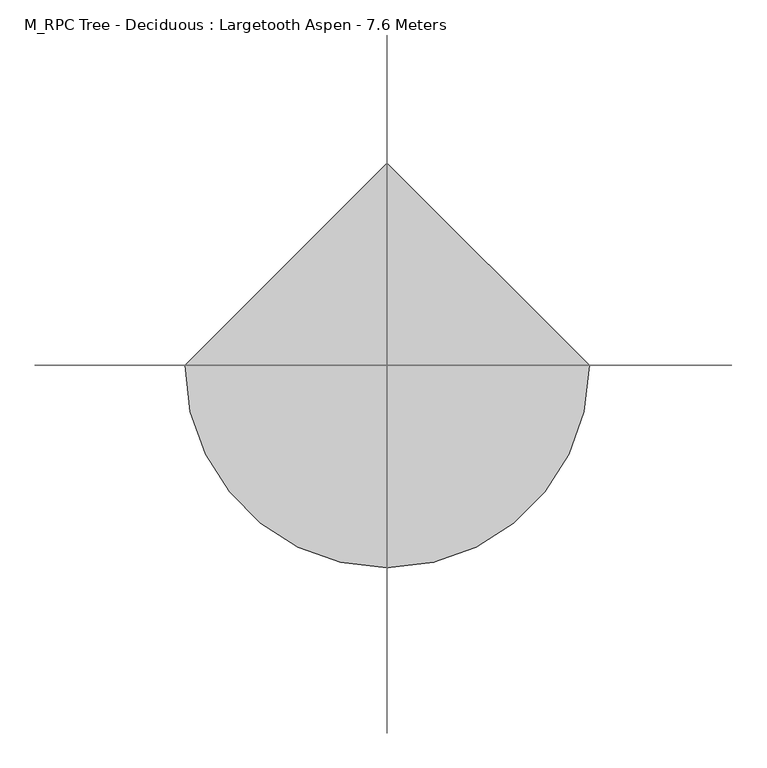
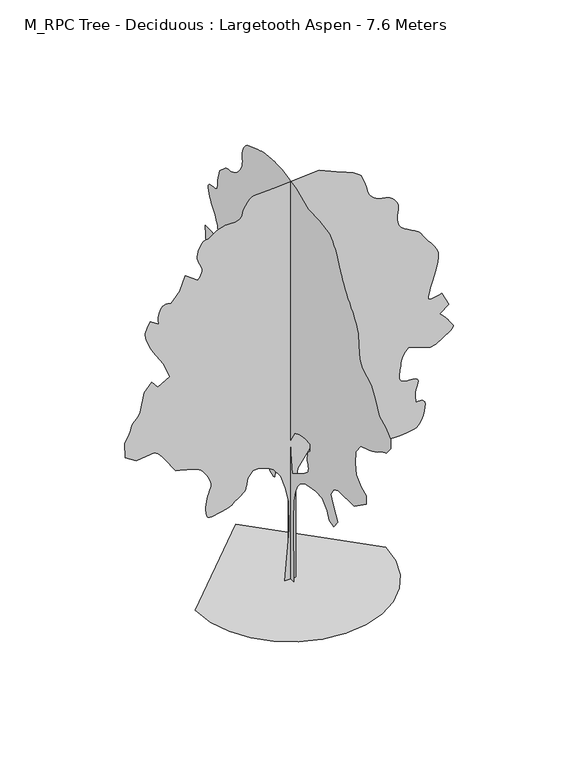
"""IFC4 building model written with IfcOpenShell, lengths in millimetres: geographic element geometry, M_RPC Tree - Deciduous : Largetooth Aspen - 7.6 Meters."""

import ifcopenshell
import ifcopenshell.guid

model = None  # the IFC model being written
_history = None  # IfcOwnerHistory: only IFC2X3 demands one
_inside = {}  # id of a spatial element -> (the spatial element, [elements in it])
_under = {}  # id of a project, library or spatial element -> (it, [spatial elements below it])
_declared = {}  # id of a project -> (the project, [libraries it declares])
_typed = {}  # id of a type object -> (the type object, [elements of that type])
_made_of = {}  # id of a material, layer set ... -> (it, [elements and type objects made of it])


def new_model(schema):
    """Start an empty IFC model of exactly this schema.

    Asked for "IFC4X3", IfcOpenShell would pick the latest addendum, in which some entities
    have other attributes; the version numbers below select the first issue.
    IFC2X3 requires an IfcOwnerHistory on every rooted entity: one is made here for all.
    """
    global model, _history
    if schema == "IFC4X3":
        model = ifcopenshell.file(schema_version=(4, 3, 0, 0))
    else:
        model = ifcopenshell.file(schema=schema)
    _inside.clear()
    _under.clear()
    _declared.clear()
    _typed.clear()
    _made_of.clear()
    _history = None
    if model.schema == "IFC2X3":
        org = make("IfcOrganization", Name="unknown")
        user = make(
            "IfcPersonAndOrganization",
            ThePerson=make("IfcPerson", FamilyName="unknown"),
            TheOrganization=org,
        )
        app = make(
            "IfcApplication",
            ApplicationDeveloper=org,
            Version="unknown",
            ApplicationFullName="unknown",
            ApplicationIdentifier="unknown",
        )
        _history = make(
            "IfcOwnerHistory",
            OwningUser=user,
            OwningApplication=app,
            ChangeAction="ADDED",
            CreationDate=0,
        )
    return model


def make(cls, **values):
    """One entity of the class cls with the attributes given. An attribute that is None is left unset."""
    return model.create_entity(
        cls, **{name: value for name, value in values.items() if value is not None}
    )


def rooted(cls, **values):
    """An entity with a GlobalId (a new one), such as an element, a storey or a relation."""
    return make(cls, GlobalId=ifcopenshell.guid.new(), OwnerHistory=_history, **values)


def si_unit(unit_type, name, prefix=None):
    """IfcSIUnit, for example si_unit("LENGTHUNIT", "METRE", prefix="MILLI")."""
    return make("IfcSIUnit", UnitType=unit_type, Prefix=prefix, Name=name)


def assignment(units):
    """IfcUnitAssignment: the units of a project."""
    return None if units is None else make("IfcUnitAssignment", Units=units)


def point(xyz):
    """IfcCartesianPoint."""
    return None if xyz is None else make("IfcCartesianPoint", Coordinates=xyz)


def direction(xyz):
    """IfcDirection."""
    return None if xyz is None else make("IfcDirection", DirectionRatios=xyz)


def frame(location, z_axis=None, x_axis=None):
    """IfcAxis2Placement3D, a coordinate frame: its origin and axes. An axis left out is left unset."""
    return make(
        "IfcAxis2Placement3D",
        Location=point(location),
        Axis=direction(z_axis),
        RefDirection=direction(x_axis),
    )


def origin():
    """The frame at (0, 0, 0) with its axes left unset."""
    return frame((0.0, 0.0, 0.0))


def place(relative_to, where):
    """IfcLocalPlacement: puts the frame where relative to a parent placement (None: the world)."""
    return make(
        "IfcLocalPlacement", PlacementRelTo=relative_to, RelativePlacement=where
    )


def context(
    kind, dimensions, precision=None, world=None, true_north=None, identifier=None
):
    """IfcGeometricRepresentationContext, for example the 3D "Model" context."""
    return make(
        "IfcGeometricRepresentationContext",
        ContextIdentifier=identifier,
        ContextType=kind,
        CoordinateSpaceDimension=dimensions,
        Precision=precision,
        WorldCoordinateSystem=world,
        TrueNorth=true_north,
    )


def project(units=None, contexts=None):
    """IfcProject with its units and contexts."""
    return rooted(
        "IfcProject",
        Name="project",
        RepresentationContexts=contexts,
        UnitsInContext=assignment(units),
    )


def spatial(cls, under=None, at=None, **own):
    """A site, building, storey or space (cls), placed at a placement, below another one or the project."""
    s = rooted(cls, ObjectPlacement=at, **own)
    if under is not None:
        _under.setdefault(under.id(), (under, []))[1].append(s)
    return s


def point_list(points):
    """IfcCartesianPointList2D or 3D."""
    cls = (
        "IfcCartesianPointList2D" if len(points[0]) == 2 else "IfcCartesianPointList3D"
    )
    return make(cls, CoordList=points)


def triangles(points, corners, closed=None, point_numbers=None):
    """IfcTriangulatedFaceSet: each triangle names its three corners, points numbered from 1."""
    return make(
        "IfcTriangulatedFaceSet",
        Coordinates=point_list(points),
        Closed=closed,
        CoordIndex=corners,
        PnIndex=point_numbers,
    )


def shape(context_of_items, identifier, shape_type, items):
    """IfcShapeRepresentation: the items that make up one representation, for example the "Body"."""
    return make(
        "IfcShapeRepresentation",
        ContextOfItems=context_of_items,
        RepresentationIdentifier=identifier,
        RepresentationType=shape_type,
        Items=items,
    )


def source(mapping_origin, context_of_items, identifier, shape_type, items):
    """IfcRepresentationMap: a shape defined once, which mapped items show again and again."""
    return make(
        "IfcRepresentationMap",
        MappingOrigin=mapping_origin,
        MappedRepresentation=shape(context_of_items, identifier, shape_type, items),
    )


def transform(
    local_origin,
    x_axis=None,
    y_axis=None,
    z_axis=None,
    scale=None,
    scale2=None,
    scale3=None,
    uniform=True,
):
    """IfcCartesianTransformationOperator3D, or its non-uniform kind. x_axis, y_axis, z_axis: its Axis1, 2, 3."""
    if uniform:
        return make(
            "IfcCartesianTransformationOperator3D",
            Axis1=direction(x_axis),
            Axis2=direction(y_axis),
            LocalOrigin=point(local_origin),
            Scale=scale,
            Axis3=direction(z_axis),
        )
    return make(
        "IfcCartesianTransformationOperator3DnonUniform",
        Axis1=direction(x_axis),
        Axis2=direction(y_axis),
        LocalOrigin=point(local_origin),
        Scale=scale,
        Axis3=direction(z_axis),
        Scale2=scale2,
        Scale3=scale3,
    )


def mapped(mapping_source, mapping_target):
    """IfcMappedItem: shows the shape of a source again, moved by a transform."""
    return make(
        "IfcMappedItem", MappingSource=mapping_source, MappingTarget=mapping_target
    )


def made_of(thing, what):
    """Note that an element or type object is made of a material, layer set ...; save() writes the relation."""
    if what is not None:
        _made_of.setdefault(what.id(), (what, []))[1].append(thing)
    return thing


def element(
    cls,
    number,
    at=None,
    inside=None,
    cuts=None,
    type_object=None,
    material=None,
    context=None,
    identifier="Body",
    shape_type=None,
    held_by="IfcProductDefinitionShape",
    body=None,
    shapes=None,
    **own,
):
    """One element of the class cls, such as IfcWall. Its Tag is "e" and its number.

    at: its placement. inside: the storey or other place that contains it. cuts: it is an
    opening in that element (IfcRelVoidsElement). A single representation is given by context,
    identifier, shape_type and body (its items); several are given by shapes. held_by: the class
    of the entity that holds the representations. save() writes the other relations.
    """
    e = rooted(cls, Tag="e%d" % number, ObjectPlacement=at, **own)
    if body is not None:
        shapes = [shape(context, identifier, shape_type, body)]
    if shapes is not None:
        e.Representation = make(held_by, Representations=shapes)
    if inside is not None:
        _inside.setdefault(inside.id(), (inside, []))[1].append(e)
    if cuts is not None:
        rooted(
            "IfcRelVoidsElement", RelatingBuildingElement=cuts, RelatedOpeningElement=e
        )
    if type_object is not None:
        _typed.setdefault(type_object.id(), (type_object, []))[1].append(e)
    return made_of(e, material)


def aggregate(whole, parts):
    """IfcRelAggregates: a whole, such as a stair, and the parts it consists of."""
    return rooted("IfcRelAggregates", RelatingObject=whole, RelatedObjects=parts)


def save(model, path):
    """Write the relations noted so far, then the file.

    IfcRelAggregates (storeys below a building ...), IfcRelContainedInSpatialStructure (elements
    in a storey), IfcRelDefinesByType, IfcRelAssociatesMaterial and IfcRelDeclares: one each for
    every whole, place, type object, material and project.
    """
    for whole, parts in _under.values():
        aggregate(whole, parts)
    for where, things in _inside.values():
        rooted(
            "IfcRelContainedInSpatialStructure",
            RelatedElements=things,
            RelatingStructure=where,
        )
    for kind, things in _typed.values():
        rooted("IfcRelDefinesByType", RelatedObjects=things, RelatingType=kind)
    for what, things in _made_of.values():
        rooted("IfcRelAssociatesMaterial", RelatedObjects=things, RelatingMaterial=what)
    for by, libraries in _declared.values():
        rooted("IfcRelDeclares", RelatingContext=by, RelatedDefinitions=libraries)
    model.write(path)


def m_rpc_tree_deciduous_largetooth_aspen_7_6_meters_a2efc43f(model_context):
    return source(origin(), model_context, "Body", "Tessellation", [
        triangles([(92.8617737, 0.000406, 0.005513), (-103.915959, 0.000406, 0.005513), (-22.8901635, 0.0003494, 949.1680813), (-34.4652064, 0.0003176, 1481.626133), (-92.3406663, 0.0003011, 1759.4311237), (-173.3674883, 0.0002866, 2002.5093098), (-300.6936918, 0.0002762, 2176.1362118), (-404.8693279, 0.0002728, 2234.0127663), (-566.9214277, 0.0002694, 2291.8891754), (-682.6743914, 0.0002694, 2291.8891754), (-763.7004049, 0.0002762, 2176.1362118), (-798.427355, 0.0002852, 2025.6589142), (-801.2950579, 0.0002863, 2008.1460297), (-806.4934324, 0.0002874, 1989.7185207), (-816.3455927, 0.0002886, 1969.4722275), (-833.1871519, 0.0002899, 1946.489764), (-859.3387533, 0.0002915, 1919.8644997), (-897.1360102, 0.0002934, 1888.6816647), (-948.9046526, 0.0002956, 1852.0320122), (-998.3097038, 0.0002977, 1817.003627), (-1032.3247061, 0.0002993, 1790.0718407), (-1058.2431822, 0.0003005, 1769.4200489), (-1083.3510246, 0.0003015, 1753.2219097), (-1114.9365967, 0.0003023, 1739.6560226), (-1160.2933485, 0.000303, 1726.8980804), (-1226.7072453, 0.0003038, 1713.1294441), (-1299.8367931, 0.0003048, 1697.5064152), (-1361.0192505, 0.0003056, 1683.0943588), (-1411.0653236, 0.0003062, 1673.9514576), (-1450.7852829, 0.0003062, 1674.1187439), (-1480.9902706, 0.0003054, 1687.6517841), (-1502.4856155, 0.0003035, 1718.5964069), (-1516.0869656, 0.0003004, 1771.0059986), (-1522.0251205, 0.0002967, 1833.4043701), (-1521.0802654, 0.0002932, 1891.7521168), (-1514.8710514, 0.00029, 1946.2541679), (-1505.0164204, 0.0002869, 1997.1108021), (-1493.1376396, 0.0002841, 2044.5246231), (-1480.8535057, 0.0002815, 2088.6983803), (-1469.7852859, 0.000279, 2129.8370029), (-1458.1775642, 0.0002769, 2165.8103886), (-1444.9485752, 0.000275, 2196.5194153), (-1432.7328964, 0.0002733, 2225.2042923), (-1424.1600185, 0.0002715, 2255.1052288), (-1421.8648098, 0.0002695, 2289.4596725), (-1428.479377, 0.000267, 2331.5079781), (-1446.6356815, 0.0002638, 2384.4900639), (-1473.3978561, 0.0002604, 2441.7913628), (-1503.3976238, 0.0002573, 2494.2338013), (-1535.6266159, 0.0002545, 2541.2094223), (-1569.0690514, 0.0002521, 2582.1226227), (-1602.7142361, 0.00025, 2616.3228607), (-1635.5487144, 0.0002484, 2643.2520309), (-1666.5642632, 0.0002473, 2662.3026123), (-1701.7269424, 0.0002464, 2677.1732162), (-1746.6125748, 0.0002455, 2692.0694), (-1799.5946606, 0.0002446, 2706.940004), (-1859.0568741, 0.0002437, 2721.8358971), (-1923.3782387, 0.0002428, 2736.706501), (-1990.9396671, 0.000242, 2751.5771049), (-2060.1197468, 0.0002411, 2766.4732887), (-2256.8962532, 0.0002238, 3055.8556252), (-2301.7818855, 0.0002202, 3116.5289566), (-2338.160479, 0.0002175, 3161.4195305), (-2367.4508423, 0.0002156, 3193.1367805), (-2391.0741096, 0.0002144, 3214.3154297), (-2410.4440029, 0.0002136, 3227.61549), (-2426.9815109, 0.0002131, 3235.6461044), (-2442.1003555, 0.0002128, 3241.041996), (-2766.1945267, 0.0002148, 3206.3353935), (-2962.9836777, 0.0002073, 3333.6607613), (-2974.5611687, 0.0001914, 3599.8884064), (-2952.3436295, 0.000189, 3639.5351143), (-2930.8609291, 0.0001867, 3678.9789276), (-2910.7717484, 0.0001843, 3718.0428223), (-2892.8103447, 0.0001821, 3756.473616), (-2877.7118477, 0.0001798, 3794.0934128), (-2866.1343567, 0.0001776, 3830.70019), (-2858.8130013, 0.0001755, 3866.1160515), (-2847.3878265, 0.0001735, 3899.5814507), (-2825.6772331, 0.0001716, 3931.2481224), (-2797.4559906, 0.0001698, 3962.0787987), (-2766.6000252, 0.0001679, 3993.137368), (-2736.9852631, 0.000166, 4025.3865623), (-2712.4120537, 0.000164, 4059.8905609), (-2696.7560326, 0.0001617, 4097.611805), (-2627.2919586, 0.000141, 4444.881015), (-2488.4021805, 0.0001321, 4595.3354942), (-2384.2239464, 0.0001396, 4468.0101265), (-2164.2953648, 0.0001327, 4583.7832924), (-2280.0483284, 0.0001155, 4873.1403397), (-2465.2501053, 9.82e-05, 5162.5226761), (-2487.5231644, 9.58e-05, 5203.6643509), (-2513.036142, 9.27e-05, 5254.9385468), (-2539.3601166, 8.93e-05, 5312.268187), (-2564.0600624, 8.58e-05, 5371.6238663), (-2584.7067673, 8.24e-05, 5428.9535065), (-2598.8934013, 7.93e-05, 5480.2277023), (-2604.1628471, 7.69e-05, 5521.3693771), (-2601.4519661, 7.48e-05, 5555.7463486), (-2593.9027176, 7.28e-05, 5589.5407974), (-2582.2746483, 7.08e-05, 5622.8038834), (-2567.4293335, 6.89e-05, 5655.6611801), (-2550.1521904, 6.69e-05, 5688.2394241), (-2531.2585762, 6.5e-05, 5720.5903564), (-2511.5516396, 6.31e-05, 5752.8651306), (-2361.0744873, 6.93e-05, 5648.6941635), (-2365.8675087, 6.73e-05, 5681.019516), (-2369.6472198, 6.54e-05, 5713.8518143), (-2371.4003105, 6.34e-05, 5747.6968414), (-2370.118412, 6.13e-05, 5783.0621246), (-2364.7857433, 5.9e-05, 5820.4540283), (-2354.391465, 5.67e-05, 5860.3794983), (-2337.9248829, 5.41e-05, 5903.344899), (-2316.394075, 5.19e-05, 5940.9141174), (-2291.8258072, 5.04e-05, 5965.7155106), (-2264.7267345, 4.95e-05, 5979.8768555), (-2235.6036575, 4.92e-05, 5985.5515091), (-2204.9604698, 4.92e-05, 5984.8422501), (-2173.3064426, 4.95e-05, 5979.8768555), (-2141.1459057, 5e-05, 5972.7831024), (-1990.6686081, 3.96e-05, 6146.4178528), (-1886.4928448, 2.44e-05, 6401.0680069), (-1666.5642632, 3.41e-05, 6239.0110382), (-1644.4939533, 3.23e-05, 6268.8284042), (-1623.9409927, 3.05e-05, 6298.823085), (-1606.4256374, 2.87e-05, 6329.2229736), (-1593.4675621, 2.69e-05, 6360.2309647), (-1586.584552, 2.5e-05, 6392.0749512), (-1587.2913403, 2.3e-05, 6424.9066681), (-1597.1131245, 2.1e-05, 6458.9545898), (-1613.1085144, 1.89e-05, 6493.7879288), (-1630.1173599, 1.68e-05, 6529.2043716), (-1646.3153538, 1.46e-05, 6565.8614365), (-1659.8813862, 1.23e-05, 6604.3428085), (-1668.993766, 9.9e-06, 6645.2304291), (-1671.8286221, 7.3e-06, 6689.1585617), (-1666.5642632, 4.4e-06, 6736.759726), (-1653.9432312, 1.5e-06, 6785.3747818), (-1636.4607227, -1.2e-06, 6830.974324), (-1614.9299149, -3.6e-06, 6871.9131042), (-1590.1616592, -5.7e-06, 6906.5691284), (-1562.9612846, -7.3e-06, 6933.3209839), (-1534.1394974, -8.3e-06, 6950.5728378), (-1504.512236, -8.7e-06, 6956.6782791), (-1471.3382435, -9.2e-06, 6965.0132355), (-1431.8891979, -1.05e-05, 6986.521225), (-1386.9707188, -1.22e-05, 7015.9078033), (-1337.3959831, -1.41e-05, 7047.9291046), (-1283.9756973, -1.59e-05, 7077.315683), (-1227.5178062, -1.72e-05, 7098.8236725), (-1168.8306908, -1.77e-05, 7107.1580475), (-1109.0314339, -1.76e-05, 7106.8289978), (-1050.4481638, -1.77e-05, 7107.2847839), (-995.7104439, -1.79e-05, 7110.8060806), (-947.4530697, -1.84e-05, 7119.5718246), (-908.3054592, -1.94e-05, 7135.8353668), (-880.9024807, -2.09e-05, 7161.8273849), (-867.8760956, -2.32e-05, 7199.7512329), (-856.9422426, -2.61e-05, 7248.5941818), (-835.6824938, -2.93e-05, 7302.6804153), (-806.5264246, -3.26e-05, 7357.4009125), (-771.9008492, -3.56e-05, 7408.0420074), (-734.2403572, -3.81e-05, 7449.9940979), (-695.9718355, -3.98e-05, 7478.5696793), (-659.5247869, -4.04e-05, 7489.1335693), (-323.8458215, -4.18e-05, 7512.2885513), (509.5693688, -4.53e-05, 7570.1751343), (926.2744205, -3.42e-05, 7384.9631836), (995.3532709, -3.26e-05, 7357.5526474), (1062.2078384, -3.09e-05, 7329.4578506), (1124.6038118, -2.92e-05, 7299.9195374), (1180.3219225, -2.73e-05, 7268.2778641), (1227.1277138, -2.52e-05, 7233.7741562), (1262.7970482, -2.29e-05, 7195.7485703), (1285.1055702, -2.04e-05, 7153.4674301), (1299.9533558, -1.79e-05, 7111.9461273), (1314.5985374, -1.58e-05, 7075.1117477), (1328.8409821, -1.37e-05, 7040.480722), (1342.4753242, -1.16e-05, 7005.6473831), (1355.2991055, -9.4e-06, 6968.1799026), (1367.1094311, -6.8e-06, 6925.6702881), (1377.7063133, -3.9e-06, 6875.662294), (1393.5345623, -8e-07, 6823.9573105), (1419.2834267, 2e-06, 6778.1292938), (1452.117905, 4.3e-06, 6738.3811386), (1489.2059029, 6.3e-06, 6704.890741), (1527.709948, 7.9e-06, 6677.9104111), (1564.7979458, 9.1e-06, 6657.5936279), (1597.6348949, 9.9e-06, 6644.1415421), (1628.0070236, 1.04e-05, 6636.0856384), (1659.1872425, 1.07e-05, 6630.6638763), (1690.5726814, 1.1e-05, 6626.230426), (1721.5527672, 1.13e-05, 6621.2144531), (1751.5195427, 1.17e-05, 6613.9439667), (1779.8675217, 1.24e-05, 6602.8481323), (1805.9861309, 1.34e-05, 6586.2799576), (1831.2638031, 1.47e-05, 6563.7586578), (1856.5388592, 1.63e-05, 6536.6015945), (1880.3977226, 1.82e-05, 6505.7959167), (1901.4218754, 2.02e-05, 6472.3560974), (1918.1949795, 2.23e-05, 6437.2948654), (1929.2986622, 2.44e-05, 6401.625531), (1933.3139694, 2.65e-05, 6366.3364059), (1929.8053173, 2.9e-05, 6325.1191544), (1922.2457497, 3.2e-05, 6273.1351181), (1915.0916805, 3.56e-05, 6213.8805954), (1912.7964718, 3.93e-05, 6150.775145), (1919.8163921, 4.31e-05, 6087.2644867), (1940.6048035, 4.67e-05, 6026.7937592), (1979.615649, 5e-05, 5972.7831024), (2034.2165314, 5.26e-05, 5927.5631882), (2096.1082478, 5.5e-05, 5888.8289246), (2161.2401733, 5.71e-05, 5853.1340103), (2225.5615379, 5.92e-05, 5817.0088898), (2285.0238968, 6.16e-05, 5777.0584213), (2335.5764797, 6.44e-05, 5729.8118866), (2373.1711327, 6.79e-05, 5671.8491455), (2411.6421856, 7.17e-05, 5607.223439), (2462.6659607, 7.56e-05, 5541.7878983), (2518.9567108, 7.96e-05, 5474.7303635), (2573.2307236, 8.38e-05, 5405.2410004), (2618.1721664, 8.81e-05, 5332.5093933), (2646.5201454, 9.27e-05, 5255.7495438), (2650.9785942, 9.76e-05, 5174.0998764), (2634.6386032, 0.0001032, 5079.7841217), (2608.190799, 0.0001097, 4970.8762344), (2575.6628426, 0.0001165, 4855.508567), (2541.0826859, 0.0001233, 4741.7367325), (2508.5622871, 0.0001295, 4637.6927925), (2482.1043091, 0.0001347, 4551.4835197), (2465.7718758, 0.0001383, 4491.1648178), (2464.9611694, 0.0001404, 4454.9635391), (2480.5538223, 0.0001417, 4433.9369156), (2509.8113388, 0.0001422, 4425.5769608), (2550.0001648, 0.0001421, 4427.3248192), (2598.3867462, 0.0001415, 4436.6727951), (2652.2453773, 0.0001407, 4451.0876129), (2708.839888, 0.0001396, 4468.0101265), (2836.1652557, 0.0001548, 4213.3596817), (2674.1332855, 0.0001624, 4086.0346046), (2698.8841003, 0.0001637, 4063.6400414), (2723.4573097, 0.0001651, 4040.7132431), (2747.6253113, 0.0001665, 4016.7987144), (2771.1852104, 0.0001681, 3991.3386406), (2793.9344032, 0.0001697, 3963.8772354), (2815.6705765, 0.0001715, 3933.8828453), (2836.1652557, 0.0001735, 3900.8482338), (2858.1037422, 0.0001754, 3868.6749069), (2881.2584335, 0.000177, 3840.554821), (2901.1702995, 0.0001786, 3814.8921432), (2913.3811821, 0.0001801, 3790.0148827), (2913.4570496, 0.0001816, 3764.3269157), (2896.9144547, 0.0001833, 3736.232119), (2859.3199471, 0.0001852, 3704.0590828), (2604.6695023, 0.0001955, 3530.4243324), (2500.4962097, 0.0001962, 3518.8471321), (2118.5182171, 0.0001886, 3646.1722092), (2091.3836815, 0.0001903, 3618.7110947), (2065.163625, 0.000192, 3590.1349319), (2040.7651142, 0.0001938, 3559.3298355), (2019.0975414, 0.0001958, 3525.1551773), (2001.0780018, 0.0001981, 3486.5726486), (1987.6134167, 0.0002008, 3442.3913338), (1979.615649, 0.0002038, 3391.5220551), (1974.0473843, 0.0002068, 3342.1474525), (1967.6684132, 0.0002092, 3301.2848305), (1961.0868382, 0.0002113, 3266.096862), (1954.9106163, 0.0002132, 3233.7206406), (1949.7477047, 0.0002151, 3201.3699989), (1946.2035896, 0.0002172, 3166.1567413), (1944.888699, 0.0002197, 3125.2941193), (1953.8643139, 0.000222, 3086.7368797), (1977.0163891, 0.0002236, 3059.0981598), (2008.6704163, 0.0002247, 3040.5542336), (2043.1591541, 0.0002254, 3029.3316628), (2074.8131813, 0.0002257, 3023.5555618), (2097.9652565, 0.0002259, 3021.4277847), (2106.9408714, 0.0002259, 3021.1237335), (2119.5973663, 0.0002258, 3022.0103073), (2151.4868443, 0.0002258, 3022.4663841), (2193.5021576, 0.000226, 3019.2997169), (2236.5307812, 0.0002266, 3009.2421913), (2271.4578644, 0.0002278, 2989.0771431), (2289.1759689, 0.0002298, 2955.5102966), (2280.5702442, 0.0002328, 2905.3758568), (2259.8146797, 0.0002362, 2847.8691925), (2246.3499493, 0.0002394, 2794.0105614), (2238.9578133, 0.0002425, 2743.191861), (2236.4270084, 0.0002453, 2694.7799904), (2237.5416206, 0.0002481, 2648.2174255), (2241.0857357, 0.0002508, 2602.8707748), (2245.8432941, 0.0002535, 2558.1066467), (2285.1910378, 0.0002532, 2562.540097), (2322.5171024, 0.0002531, 2563.730722), (2355.7899261, 0.0002535, 2558.4106979), (2382.9903008, 0.0002544, 2543.4133575), (2402.0916058, 0.000256, 2515.4278564), (2411.0672207, 0.0002587, 2471.2540993), (2407.8954666, 0.0002625, 2407.6395229), (2395.1731327, 0.0002668, 2334.9507912), (2376.9836906, 0.0002708, 2266.9155544), (2353.5301804, 0.0002745, 2205.3632069), (2325.0124443, 0.0002777, 2152.110062), (2291.6383186, 0.0002803, 2108.9801365), (2253.6054657, 0.0002821, 2077.7999176), (2211.1189602, 0.0002832, 2060.3858643), (2171.2620907, 0.0002837, 2051.7801395), (2137.4826118, 0.000284, 2045.4011684), (2104.5113686, 0.0002843, 2040.64361), (2067.0864727, 0.0002845, 2036.8967457), (2019.9412399, 0.0002847, 2033.5578506), (1957.8137821, 0.000285, 2030.0137356), (1875.4374149, 0.0002852, 2025.6589142), (1785.9069786, 0.0002851, 2027.1105698), (1704.880965, 0.0002844, 2040.1039627), (1630.9405655, 0.000283, 2062.7139198), (1562.6724941, 0.0002812, 2093.0175934), (1498.6551807, 0.0002791, 2129.0947517), (1437.4727234, 0.0002767, 2169.0176056), (1377.7063133, 0.0002742, 2210.8631618), (1123.0508543, 0.0002597, 2453.9412025), (856.8231365, 0.0002528, 2569.6841377), (544.2937391, 0.0002542, 2546.5547356), (393.8164052, 0.0002611, 2430.7917435), (289.6407691, 0.00027, 2280.3144459), (127.5871523, 0.0002838, 2048.8109894), (92.8617737, 0.0003011, 1759.4311237), (92.8617737, 0.0003383, 1134.3723289), (-0.0023646, 90.6053344, 1.1e-05), (-0.0023646, -94.5971056, 0.0), (-0.0023646, -83.0220672, 1157.5168465), (-0.0023646, -94.5971056, 1527.9227257), (-0.0023646, -140.8980313, 1724.6992321), (-0.0023646, -210.3490428, 1875.1765297), (-0.0023646, -302.9508941, 1990.9294933), (-0.0023646, -441.8534077, 2071.9555069), (-0.0023646, -557.6038279, 2095.1051113), (-0.0023646, -789.1072117, 2141.4067909), (-0.0023646, -985.8861889, 2129.8320614), (-0.0023646, -1136.3635592, 1979.3546185), (-0.0023646, -1205.8147705, 1840.4521957), (-0.0023646, -1333.1399929, 1794.1505161), (-0.0023646, -1472.042561, 1967.7774181), (-0.0023646, -1321.5652634, 2199.2832001), (-0.0023646, -1252.1139793, 2361.3353725), (-0.0023646, -1333.1399929, 2500.2354698), (-0.0023646, -1483.6172905, 2569.6841377), (-0.0023646, -1969.7736626, 2569.6841377), (-0.0023646, -2351.7542713, 2835.9117828), (-0.0023646, -2351.7542713, 2997.9690422), (-0.0023646, -2189.7022442, 3067.4075363), (-0.0023646, -2039.2249466, 3206.3101044), (-0.0023646, -2004.5004673, 3403.0992554), (-0.0023646, -2027.6500717, 3634.5950089), (-0.0023646, -2178.1273693, 3831.3841599), (-0.0023646, -2444.3551598, 3923.9773453), (-0.0023646, -2488.9367409, 3941.4068047), (-0.0023646, -2533.110498, 3959.1147354), (-0.0023646, -2576.4735489, 3977.4307686), (-0.0023646, -2618.6279526, 3996.6839539), (-0.0023646, -2659.1612343, 4017.1280548), (-0.0023646, -2697.6678955, 4039.0918304), (-0.0023646, -2733.7427284, 4062.8799133), (-0.0023646, -2768.4493309, 4086.3386559), (-0.0023646, -2803.1812225, 4107.3652794), (-0.0023646, -2837.9131142, 4126.3652824), (-0.0023646, -2872.6450058, 4143.7438728), (-0.0023646, -2907.351899, 4159.9065491), (-0.0023646, -2942.0837906, 4175.258519), (-0.0023646, -2976.8156822, 4190.2052811), (-0.0023646, -3104.1407593, 4352.2622498), (-0.0023646, -3104.1407593, 4514.3195091), (-0.0023646, -2953.6609909, 4653.2220772), (-0.0023646, -2756.8971291, 4757.3924629), (-0.0023646, -2629.5467628, 5000.4657074), (-0.0023646, -2502.234185, 5185.6776581), (-0.0023646, -2224.4290489, 5336.1574265), (-0.0023646, -2143.4030354, 5463.4827942), (-0.0023646, -2120.2509602, 5718.1329483), (-0.0023646, -2097.1013557, 5926.4743011), (-0.0023646, -2072.264645, 5978.4327576), (-0.0023646, -2047.225185, 6029.4540619), (-0.0023646, -2021.7779011, 6078.651059), (-0.0023646, -1995.7251308, 6125.1127579), (-0.0023646, -1968.8641251, 6167.9514221), (-0.0023646, -1940.9873383, 6206.2043198), (-0.0023646, -1911.8997242, 6239.0110382), (-0.0023646, -1875.8225658, 6277.7964615), (-0.0023646, -1830.2327614, 6330.9455429), (-0.0023646, -1779.7788643, 6393.0121033), (-0.0023646, -1729.1274502, 6458.4988037), (-0.0023646, -1682.9270725, 6521.9838821), (-0.0023646, -1645.83922, 6577.9705811), (-0.0023646, -1622.5198586, 6620.9865601), (-0.0023646, -1605.6807701, 6657.1372604), (-0.0023646, -1585.6016178, 6696.1255783), (-0.0023646, -1563.2930958, 6737.9253525), (-0.0023646, -1539.7736012, 6782.5877426), (-0.0023646, -1516.0490318, 6830.0627518), (-0.0023646, -1493.1350235, 6880.3742157), (-0.0023646, -1472.042561, 6933.5238785), (-0.0023646, -1448.8245014, 6986.749118), (-0.0023646, -1419.5316673, 7037.5425293), (-0.0023646, -1385.1770782, 7086.3087387), (-0.0023646, -1346.7743351, 7133.4541168), (-0.0023646, -1305.3316612, 7179.3832901), (-0.0023646, -1261.8673084, 7224.5020477), (-0.0023646, -1217.3895727, 7269.2155975), (-0.0023646, -893.2828297, 7327.0766006), (-0.0023646, -546.029062, 7338.653801), (-0.0023646, -175.623419, 7500.711351), (-0.0023646, 264.2314734, 7593.3045364), (-0.0023646, 323.6937959, 7595.7363647), (-0.0023646, 382.7508016, 7597.8641418), (-0.0023646, 440.9996807, 7599.3843979), (-0.0023646, 498.0300296, 7599.9925003), (-0.0023646, 553.4441254, 7599.3843979), (-0.0023646, 606.831528, 7597.2566208), (-0.0023646, 657.7895004, 7593.3045364), (-0.0023646, 706.7891258, 7588.2379852), (-0.0023646, 754.9781902, 7582.5883301), (-0.0023646, 802.9670488, 7575.6974716), (-0.0023646, 851.3612606, 7566.9828873), (-0.0023646, 900.7663118, 7555.8620544), (-0.0023646, 951.7900869, 7541.6751297), (-0.0023646, 1005.0432318, 7523.8657516), (-0.0023646, 1340.7248497, 7408.1181656), (-0.0023646, 1370.3545818, 7383.1138779), (-0.0023646, 1399.173753, 7356.8683868), (-0.0023646, 1426.3741276, 7328.2166473), (-0.0023646, 1451.1425285, 7295.9418732), (-0.0023646, 1472.6733364, 7258.7778625), (-0.0023646, 1490.1558449, 7215.5595703), (-0.0023646, 1502.7768768, 7165.019632), (-0.0023646, 1507.1292274, 7116.7342072), (-0.0023646, 1503.584967, 7077.7714691), (-0.0023646, 1497.0060081, 7043.2421814), (-0.0023646, 1492.2458336, 7008.3076859), (-0.0023646, 1494.1711521, 6968.128743), (-0.0023646, 1507.6358826, 6917.7916992), (-0.0023646, 1537.5012108, 6852.5078934), (-0.0023646, 1578.4019119, 6786.1851974), (-0.0023646, 1620.9238804, 6734.4546341), (-0.0023646, 1663.8485859, 6694.8587952), (-0.0023646, 1705.9652012, 6664.9908508), (-0.0023646, 1746.0576668, 6642.4189728), (-0.0023646, 1782.9075977, 6624.7107513), (-0.0023646, 1815.3063469, 6609.4093597), (-0.0023646, 1845.0703732, 6598.3135254), (-0.0023646, 1874.8345448, 6592.8923447), (-0.0023646, 1904.598571, 6590.2826202), (-0.0023646, 1934.3652134, 6587.6984756), (-0.0023646, 1964.129385, 6582.2522964), (-0.0023646, 1993.8934113, 6571.1558807), (-0.0023646, 2023.6575829, 6551.5483566), (-0.0023646, 2197.2869556, 6401.0680069), (-0.0023646, 2266.7357689, 6181.1500351), (-0.0023646, 2264.4760231, 6146.5445892), (-0.0023646, 2263.5310226, 6112.7751389), (-0.0023646, 2265.2182743, 6080.6021027), (-0.0023646, 2270.8549942, 6050.8858932), (-0.0023646, 2281.7533115, 6024.3875107), (-0.0023646, 2299.23582, 6001.9417877), (-0.0023646, 2324.612178, 5984.3608841), (-0.0023646, 2359.9116222, 5974.3033585), (-0.0023646, 2402.9047829, 5970.5285889), (-0.0023646, 2448.5301956, 5967.9700241), (-0.0023646, 2491.7284309, 5961.5605316), (-0.0023646, 2527.4306122, 5946.2341415), (-0.0023646, 2550.5826874, 5916.92314), (-0.0023646, 2556.1053154, 5868.6127167), (-0.0023646, 2547.4413094, 5812.448703), (-0.0023646, 2532.0893394, 5762.3651321), (-0.0023646, 2511.1641632, 5717.3475311), (-0.0023646, 2485.7878052, 5676.3837524), (-0.0023646, 2457.0700813, 5638.4599045), (-0.0023646, 2426.1228424, 5602.562677), (-0.0023646, 2394.0634621, 5567.6531799), (-0.0023646, 2369.3609001, 5525.4981949), (-0.0023646, 2345.2664406, 5483.4705276), (-0.0023646, 2322.3854244, 5441.6201752), (-0.0023646, 2301.3284248, 5400.0732925), (-0.0023646, 2282.698312, 5358.9321991), (-0.0023646, 2267.1081299, 5318.2974701), (-0.0023646, 2255.160894, 5278.2708435), (-0.0023646, 2248.95168, 5240.6254669), (-0.0023646, 2249.4254883, 5206.6025436), (-0.0023646, 2255.4649452, 5175.6201324), (-0.0023646, 2265.9605255, 5147.0695496), (-0.0023646, 2279.797617, 5120.3426926), (-0.0023646, 2295.861462, 5094.8320404), (-0.0023646, 2313.0374485, 5069.9294907), (-0.0023646, 2463.5147461, 5093.0844727), (-0.0023646, 2648.7240807, 5093.0844727), (-0.0023646, 2625.5693893, 4757.3924629), (-0.0023646, 2417.2130665, 4398.5716324), (-0.0023646, 2409.7574169, 4356.4422272), (-0.0023646, 2402.1979946, 4314.642453), (-0.0023646, 2394.4358231, 4273.4252014), (-0.0023646, 2386.3697456, 4233.1451019), (-0.0023646, 2377.898315, 4194.0559181), (-0.0023646, 2368.9227001, 4156.486409), (-0.0023646, 2359.3391281, 4120.7664963), (-0.0023646, 2344.9953815, 4082.1586784), (-0.0023646, 2323.9712288, 4037.2681046), (-0.0023646, 2299.5044083, 3988.3492882), (-0.0023646, 2274.8373093, 3937.5814568), (-0.0023646, 2253.2051994, 3887.2441223), (-0.0023646, 2237.8507587, 3839.5162216), (-0.0023646, 2232.0114349, 3796.6522682), (-0.0023646, 2236.7360012, 3758.6522621), (-0.0023646, 2249.9651356, 3723.6921867), (-0.0023646, 2270.279884, 3691.2656776), (-0.0023646, 2296.2641991, 3660.865789), (-0.0023646, 2326.5020336, 3631.9602859), (-0.0023646, 2359.5747242, 3604.0936729), (-0.0023646, 2394.0634621, 3576.7337151), (-0.0023646, 2706.5853745, 3646.1722092), (-0.0023646, 2723.8372284, 3596.6458717), (-0.0023646, 2740.3798233, 3547.4991623), (-0.0023646, 2755.5039001, 3499.1884483), (-0.0023646, 2768.4746201, 3452.0686501), (-0.0023646, 2778.6333023, 3406.5699738), (-0.0023646, 2785.245108, 3363.0979179), (-0.0023646, 2787.6266487, 3322.0832703), (-0.0023646, 2774.199852, 3282.9940865), (-0.0023646, 2739.6958534, 3244.7153183), (-0.0023646, 2692.8545265, 3206.6647339), (-0.0023646, 2642.3654572, 3168.1833618), (-0.0023646, 2596.9426483, 3128.7142593), (-0.0023646, 2565.3015564, 3087.5981644), (-0.0023646, 2556.1053154, 3044.2784248), (-0.0023646, 2564.4399811, 3002.6556747), (-0.0023646, 2578.8547989, 2966.5049744), (-0.0023646, 2598.3361679, 2934.9397499), (-0.0023646, 2621.8454887, 2906.9969788), (-0.0023646, 2648.4200294, 2881.7903778), (-0.0023646, 2676.9959015, 2858.3825043), (-0.0023646, 2706.5853745, 2835.9117828), (-0.0023646, 2776.0491577, 2604.4160294), (-0.0023646, 2709.3974121, 2602.1106468), (-0.0023646, 2644.670549, 2600.945311), (-0.0023646, 2583.7946136, 2601.984201), (-0.0023646, 2528.6796638, 2606.3667824), (-0.0023646, 2481.2656975, 2615.2081032), (-0.0023646, 2443.468586, 2629.6226303), (-0.0023646, 2417.2130665, 2650.725412), (-0.0023646, 2391.9710026, 2676.8694557), (-0.0023646, 2357.0109272, 2705.4453278), (-0.0023646, 2313.9494568, 2736.0478203), (-0.0023646, 2264.407568, 2768.2973053), (-0.0023646, 2210.0068188, 2801.7371246), (-0.0023646, 2152.3684765, 2835.987941), (-0.0023646, 2093.1088669, 2870.6436745), (-0.0023646, 2090.6463718, 2833.3785072), (-0.0023646, 2088.2828533, 2795.8345779), (-0.0023646, 2086.1244095, 2757.6572571), (-0.0023646, 2084.2675461, 2718.5680733), (-0.0023646, 2082.8158905, 2678.2879738), (-0.0023646, 2081.8710354, 2636.4626198), (-0.0023646, 2081.533992, 2592.838829), (-0.0023646, 2079.9481876, 2547.390731), (-0.0023646, 2074.514217, 2502.7332825), (-0.0023646, 2064.2212406, 2462.5418404), (-0.0023646, 2048.0560936, 2430.4471424), (-0.0023646, 2025.0077911, 2410.0994019), (-0.0023646, 1994.0631683, 2405.1366234), (-0.0023646, 1954.2062988, 2419.2093109), (-0.0023646, 1909.2219807, 2445.3635284), (-0.0023646, 1863.6321762, 2473.9469582), (-0.0023646, 1817.5331005, 2504.5546829), (-0.0023646, 1771.028817, 2536.7762627), (-0.0023646, 1724.222953, 2570.216082), (-0.0023646, 1677.2144852, 2604.4921875), (-0.0023646, 1630.1020992, 2639.147921), (-0.0023646, 1352.2995792, 2720.1639061), (-0.0023646, 1074.4945158, 2627.5707207), (-0.0023646, 900.8676138, 2419.2093109), (-0.0023646, 923.2419748, 2389.5794334), (-0.0023646, 945.9203871, 2360.7602623), (-0.0023646, 969.204213, 2333.5598877), (-0.0023646, 993.4000471, 2308.7914867), (-0.0023646, 1018.8119408, 2287.2608242), (-0.0023646, 1045.7412563, 2269.7783157), (-0.0023646, 1074.4945158, 2257.1571384), (-0.0023646, 1101.897567, 2244.8731499), (-0.0023646, 1125.0471714, 2228.3379673), (-0.0023646, 1144.6551315, 2208.258815), (-0.0023646, 1161.4257648, 2185.344952), (-0.0023646, 1176.07349, 2160.305492), (-0.0023646, 1189.3025517, 2133.8473686), (-0.0023646, 1201.8222816, 2106.6798409), (-0.0023646, 1169.4919149, 2099.1888737), (-0.0023646, 1136.6573639, 2091.3937099), (-0.0023646, 1102.8070318, 2082.9907345), (-0.0023646, 1067.4417486, 2073.6756054), (-0.0023646, 1030.0497723, 2063.1471783), (-0.0023646, 990.1269911, 2051.0986404), (-0.0023646, 947.16675, 2037.2285568), (-0.0023646, 904.2091249, 2020.3237747), (-0.0023646, 864.2863438, 1999.7708141), (-0.0023646, 826.8943674, 1976.1830097), (-0.0023646, 791.5265408, 1950.1630863), (-0.0023646, 757.6786795, 1922.3217625), (-0.0023646, 724.8442011, 1893.2645245), (-0.0023646, 692.5138344, 1863.6018002), (-0.0023646, 692.5138344, 1701.5496277), (-0.0023646, 650.5998957, 1674.7216141), (-0.0023646, 610.2059223, 1650.6246838), (-0.0023646, 572.8469018, 1631.9970417), (-0.0023646, 540.0453429, 1621.5699165), (-0.0023646, 513.3187039, 1622.0765717), (-0.0023646, 494.1844431, 1636.2505611), (-0.0023646, 484.160055, 1666.8252937), (-0.0023646, 479.2682024, 1701.4811726), (-0.0023646, 474.7791232, 1728.6487003), (-0.0023646, 471.100714, 1752.1706657), (-0.0023646, 468.638328, 1775.8927643), (-0.0023646, 467.7947385, 1803.6682491), (-0.0023646, 468.9752624, 1839.3374382), (-0.0023646, 472.5852528, 1886.7512592), (-0.0023646, 475.5213744, 1938.6212036), (-0.0023646, 474.8120427, 1985.6298168), (-0.0023646, 471.0677945, 2028.5899853), (-0.0023646, 464.8915363, 2068.3100899), (-0.0023646, 456.893805, 2105.6006916), (-0.0023646, 447.6800869, 2141.2724968), (-0.0023646, 437.8608825, 2176.1311249), (-0.0023646, 241.0823958, 2187.7059998), (-0.0023646, 136.90626, 1990.9294933), (-0.0023646, 79.030296, 1655.2479481), (-0.0023646, 79.030296, 1226.9681305), (-0.0023646, 79.030296, 590.3344608), (-0.0022449, -48.2969385, 2025.6538273), (-0.0022449, -1.9959556, 2396.0597065), (-0.0022449, 9.5791312, 2615.9935204), (-0.0022449, -129.3229929, 2835.9117828), (-0.0022449, -279.801326, 2905.3758568), (-0.0022449, -453.4282099, 2928.5049683), (-0.0022449, -615.4803097, 2928.5049683), (-0.0022449, -615.4803097, 2789.62798), (-0.0022449, -534.4542598, 2720.1639061), (-0.0022449, -511.3046917, 2558.1066467), (-0.0022449, -521.1568156, 2548.0241226), (-0.0022449, -530.6061298, 2536.9279976), (-0.0022449, -539.2448104, 2523.7927528), (-0.0022449, -546.6699749, 2507.6277512), (-0.0022449, -552.4738358, 2487.4115433), (-0.0022449, -556.2535832, 2462.1366325), (-0.0022449, -557.6038279, 2430.7840405), (-0.0022449, -554.2294335, 2398.4207542), (-0.0022449, -544.7801193, 2370.3109875), (-0.0022449, -530.2691955, 2345.7427197), (-0.0022449, -511.7075014, 2324.0093079), (-0.0022449, -490.1108545, 2304.4038185), (-0.0022449, -466.4875508, 2286.2145218), (-0.0022449, -441.8534077, 2268.7320133), (-1707.3661331, 0.0, 0.0031185), (-1662.2297894, -391.2146745, 0.0030952), (-1533.678479, -750.4840605, 0.0030738), (-1332.01012, -1067.5126745, 0.0030549), (-1067.5126745, -1332.01012, 0.0030391), (-750.4840605, -1533.678479, 0.0030271), (-391.2146745, -1662.2297894, 0.0030194), (7.48e-05, -1707.3661331, 0.0030167), (391.2146745, -1662.2297894, 0.0030194), (750.4840605, -1533.678479, 0.0030271), (1067.5126745, -1332.01012, 0.0030391), (1332.01012, -1067.5126745, 0.0030549), (1533.678479, -750.4840605, 0.0030738), (1662.2297894, -391.2146745, 0.0030952), (1707.3661331, 0.0001493, 0.0031185), (-0.0002245, 1707.3661331, 0.0032203)], [[122, 123, 124], [87, 88, 89], [1, 2, 3], [329, 1, 3], [329, 3, 4], [328, 329, 4], [328, 4, 5], [105, 106, 107], [327, 328, 5], [327, 5, 6], [104, 105, 107], [238, 239, 240], [238, 240, 241], [237, 238, 241], [236, 237, 241], [103, 104, 107], [86, 87, 89], [235, 236, 241], [102, 103, 107], [101, 102, 107], [100, 101, 107], [99, 100, 107], [98, 99, 107], [97, 98, 107], [96, 97, 107], [327, 6, 7], [326, 327, 7], [95, 96, 107], [70, 71, 72], [69, 70, 72], [69, 72, 73], [69, 73, 74], [69, 74, 75], [69, 75, 76], [69, 76, 77], [69, 77, 78], [94, 95, 107], [234, 235, 241], [93, 94, 107], [69, 78, 79], [69, 79, 80], [69, 80, 81], [69, 81, 82], [69, 82, 83], [69, 83, 84], [69, 84, 85], [68, 69, 85], [325, 326, 7], [325, 7, 8], [67, 68, 85], [92, 93, 107], [91, 92, 107], [60, 61, 62], [67, 85, 86], [67, 86, 89], [67, 89, 90], [66, 67, 90], [65, 66, 90], [64, 65, 90], [63, 64, 90], [62, 63, 90], [60, 62, 90], [59, 60, 90], [58, 59, 90], [57, 58, 90], [56, 57, 90], [55, 56, 90], [54, 55, 90], [53, 54, 90], [284, 285, 286], [283, 284, 286], [282, 283, 286], [282, 286, 287], [281, 282, 287], [280, 281, 287], [279, 280, 287], [279, 287, 288], [278, 279, 288], [277, 278, 288], [277, 288, 289], [276, 277, 289], [275, 276, 289], [275, 289, 290], [52, 53, 90], [325, 8, 9], [121, 122, 124], [275, 290, 291], [30, 31, 32], [29, 30, 32], [29, 32, 33], [28, 29, 33], [28, 33, 34], [27, 28, 34], [27, 34, 35], [27, 35, 36], [26, 27, 36], [26, 36, 37], [26, 37, 38], [25, 26, 38], [25, 38, 39], [24, 25, 39], [23, 24, 39], [22, 23, 39], [21, 22, 39], [20, 21, 39], [20, 39, 40], [20, 40, 41], [20, 41, 42], [19, 20, 42], [19, 42, 43], [18, 19, 43], [18, 43, 44], [17, 18, 44], [16, 17, 44], [15, 16, 44], [14, 15, 44], [13, 14, 44], [12, 13, 44], [11, 12, 44], [11, 44, 45], [11, 45, 46], [10, 11, 46], [10, 46, 47], [10, 47, 48], [10, 48, 49], [10, 49, 50], [10, 50, 51], [252, 253, 254], [251, 252, 254], [251, 254, 255], [250, 251, 255], [249, 250, 255], [249, 255, 256], [248, 249, 256], [247, 248, 256], [246, 247, 256], [245, 246, 256], [245, 256, 257], [245, 257, 258], [244, 245, 258], [243, 244, 258], [242, 243, 258], [241, 242, 258], [234, 241, 258], [233, 234, 258], [274, 275, 291], [324, 325, 9], [51, 52, 90], [10, 51, 90], [9, 10, 90], [324, 9, 90], [323, 324, 90], [323, 90, 91], [323, 91, 107], [323, 107, 108], [323, 108, 109], [323, 109, 110], [323, 110, 111], [323, 111, 112], [323, 112, 113], [323, 113, 114], [323, 114, 115], [323, 115, 116], [323, 116, 117], [323, 117, 118], [323, 118, 119], [323, 119, 120], [323, 120, 121], [323, 121, 124], [323, 124, 125], [323, 125, 126], [323, 126, 127], [323, 127, 128], [323, 128, 129], [322, 323, 129], [322, 129, 130], [167, 168, 169], [274, 291, 292], [296, 297, 298], [296, 298, 299], [295, 296, 299], [294, 295, 299], [294, 299, 300], [293, 294, 300], [293, 300, 301], [293, 301, 302], [293, 302, 303], [293, 303, 304], [293, 304, 305], [293, 305, 306], [293, 306, 307], [293, 307, 308], [293, 308, 309], [293, 309, 310], [293, 310, 311], [293, 311, 312], [293, 312, 313], [293, 313, 314], [293, 314, 315], [293, 315, 316], [293, 316, 317], [293, 317, 318], [293, 318, 319], [292, 293, 319], [274, 292, 319], [274, 319, 320], [274, 320, 321], [274, 321, 322], [273, 274, 322], [273, 322, 130], [272, 273, 130], [271, 272, 130], [270, 271, 130], [269, 270, 130], [268, 269, 130], [267, 268, 130], [266, 267, 130], [265, 266, 130], [264, 265, 130], [263, 264, 130], [262, 263, 130], [261, 262, 130], [260, 261, 130], [259, 260, 130], [258, 259, 130], [233, 258, 130], [232, 233, 130], [231, 232, 130], [230, 231, 130], [229, 230, 130], [228, 229, 130], [227, 228, 130], [226, 227, 130], [225, 226, 130], [224, 225, 130], [223, 224, 130], [222, 223, 130], [221, 222, 130], [220, 221, 130], [219, 220, 130], [218, 219, 130], [217, 218, 130], [216, 217, 130], [215, 216, 130], [214, 215, 130], [213, 214, 130], [212, 213, 130], [211, 212, 130], [210, 211, 130], [209, 210, 130], [208, 209, 130], [207, 208, 130], [206, 207, 130], [205, 206, 130], [204, 205, 130], [203, 204, 130], [202, 203, 130], [201, 202, 130], [200, 201, 130], [199, 200, 130], [198, 199, 130], [197, 198, 130], [196, 197, 130], [195, 196, 130], [194, 195, 130], [193, 194, 130], [192, 193, 130], [191, 192, 130], [190, 191, 130], [189, 190, 130], [188, 189, 130], [187, 188, 130], [186, 187, 130], [185, 186, 130], [184, 185, 130], [183, 184, 130], [182, 183, 130], [181, 182, 130], [180, 181, 130], [179, 180, 130], [178, 179, 130], [177, 178, 130], [176, 177, 130], [175, 176, 130], [174, 175, 130], [173, 174, 130], [172, 173, 130], [171, 172, 130], [170, 171, 130], [169, 170, 130], [167, 169, 130], [167, 130, 131], [167, 131, 132], [167, 132, 133], [167, 133, 134], [167, 134, 135], [167, 135, 136], [164, 165, 166], [164, 166, 167], [163, 164, 167], [162, 163, 167], [161, 162, 167], [160, 161, 167], [159, 160, 167], [158, 159, 167], [143, 144, 145], [142, 143, 145], [141, 142, 145], [140, 141, 145], [140, 145, 146], [139, 140, 146], [138, 139, 146], [137, 138, 146], [136, 137, 146], [136, 146, 147], [136, 147, 148], [136, 148, 149], [136, 149, 150], [136, 150, 151], [136, 151, 152], [136, 152, 153], [136, 153, 154], [136, 154, 155], [136, 155, 156], [157, 158, 167], [157, 167, 136], [157, 136, 156], [634, 330, 635], [633, 634, 635], [632, 633, 635], [631, 632, 635], [540, 541, 542], [592, 593, 594], [494, 495, 496], [635, 330, 331], [635, 331, 332], [635, 332, 333], [635, 333, 334], [635, 334, 335], [658, 635, 335], [658, 335, 336], [658, 336, 337], [658, 337, 338], [540, 542, 543], [657, 658, 338], [631, 635, 636], [630, 631, 636], [518, 519, 520], [656, 657, 338], [656, 338, 339], [655, 656, 339], [654, 655, 339], [653, 654, 339], [540, 543, 544], [539, 540, 544], [518, 520, 521], [539, 544, 545], [538, 539, 545], [538, 545, 546], [538, 546, 547], [538, 547, 548], [537, 538, 548], [537, 548, 549], [536, 537, 549], [536, 549, 550], [536, 550, 551], [535, 536, 551], [535, 551, 552], [534, 535, 552], [493, 494, 496], [493, 496, 497], [343, 344, 345], [342, 343, 345], [341, 342, 345], [340, 341, 345], [340, 345, 346], [534, 552, 553], [533, 534, 553], [518, 521, 522], [350, 351, 352], [349, 350, 352], [349, 352, 353], [348, 349, 353], [533, 553, 554], [652, 653, 339], [518, 522, 523], [518, 523, 524], [533, 554, 555], [532, 533, 555], [518, 524, 525], [518, 525, 526], [518, 526, 527], [518, 527, 528], [518, 528, 529], [518, 529, 530], [518, 530, 531], [518, 531, 532], [518, 532, 555], [517, 518, 555], [516, 517, 555], [515, 516, 555], [607, 608, 609], [591, 592, 594], [591, 594, 595], [590, 591, 595], [590, 595, 596], [589, 590, 596], [588, 589, 596], [588, 596, 597], [587, 588, 597], [586, 587, 597], [586, 597, 598], [585, 586, 598], [585, 598, 599], [584, 585, 599], [584, 599, 600], [583, 584, 600], [583, 600, 601], [582, 583, 601], [514, 515, 555], [643, 644, 645], [630, 636, 637], [629, 630, 637], [581, 582, 601], [581, 601, 602], [348, 353, 354], [580, 581, 602], [580, 602, 603], [579, 580, 603], [651, 652, 339], [651, 339, 340], [651, 340, 346], [650, 651, 346], [649, 650, 346], [649, 346, 347], [648, 649, 347], [647, 648, 347], [646, 647, 347], [372, 373, 374], [371, 372, 374], [370, 371, 374], [369, 370, 374], [369, 374, 375], [368, 369, 375], [367, 368, 375], [366, 367, 375], [365, 366, 375], [364, 365, 375], [363, 364, 375], [362, 363, 375], [361, 362, 375], [360, 361, 375], [359, 360, 375], [358, 359, 375], [357, 358, 375], [356, 357, 375], [356, 375, 376], [356, 376, 377], [356, 377, 378], [645, 646, 347], [643, 645, 347], [642, 643, 347], [641, 642, 347], [641, 347, 348], [641, 348, 354], [641, 354, 355], [607, 609, 610], [513, 514, 555], [579, 603, 604], [607, 610, 611], [607, 611, 612], [607, 612, 613], [607, 613, 614], [607, 614, 615], [607, 615, 616], [607, 616, 617], [607, 617, 618], [607, 618, 619], [607, 619, 620], [607, 620, 621], [607, 621, 622], [607, 622, 623], [607, 623, 624], [606, 607, 624], [606, 624, 625], [605, 606, 625], [605, 625, 626], [604, 605, 626], [579, 604, 626], [579, 626, 627], [579, 627, 628], [579, 628, 629], [579, 629, 637], [578, 579, 637], [578, 637, 638], [355, 356, 378], [641, 355, 378], [641, 378, 379], [640, 641, 379], [639, 640, 379], [639, 379, 380], [639, 380, 381], [639, 381, 382], [639, 382, 383], [639, 383, 384], [639, 384, 385], [639, 385, 386], [639, 386, 387], [639, 387, 388], [639, 388, 389], [639, 389, 390], [639, 390, 391], [639, 391, 392], [639, 392, 393], [639, 393, 394], [639, 394, 395], [638, 639, 395], [578, 638, 395], [577, 578, 395], [577, 395, 396], [577, 396, 397], [577, 397, 398], [577, 398, 399], [577, 399, 400], [577, 400, 401], [577, 401, 402], [577, 402, 403], [577, 403, 404], [577, 404, 405], [577, 405, 406], [577, 406, 407], [577, 407, 408], [577, 408, 409], [577, 409, 410], [577, 410, 411], [577, 411, 412], [577, 412, 413], [577, 413, 414], [577, 414, 415], [577, 415, 416], [577, 416, 417], [577, 417, 418], [577, 418, 419], [577, 419, 420], [577, 420, 421], [577, 421, 422], [577, 422, 423], [577, 423, 424], [577, 424, 425], [577, 425, 426], [577, 426, 427], [577, 427, 428], [577, 428, 429], [577, 429, 430], [577, 430, 431], [577, 431, 432], [577, 432, 433], [577, 433, 434], [566, 567, 568], [566, 568, 569], [565, 566, 569], [564, 565, 569], [564, 569, 570], [563, 564, 570], [563, 570, 571], [562, 563, 571], [562, 571, 572], [561, 562, 572], [560, 561, 572], [560, 572, 573], [559, 560, 573], [559, 573, 574], [558, 559, 574], [558, 574, 575], [557, 558, 575], [556, 557, 575], [556, 575, 576], [555, 556, 576], [513, 555, 576], [513, 576, 577], [512, 513, 577], [511, 512, 577], [470, 471, 472], [469, 470, 472], [468, 469, 472], [468, 472, 473], [467, 468, 473], [467, 473, 474], [467, 474, 475], [466, 467, 475], [466, 475, 476], [466, 476, 477], [465, 466, 477], [465, 477, 478], [465, 478, 479], [464, 465, 479], [464, 479, 480], [464, 480, 481], [464, 481, 482], [463, 464, 482], [456, 457, 458], [456, 458, 459], [456, 459, 460], [510, 511, 577], [463, 482, 483], [455, 456, 460], [454, 455, 460], [453, 454, 460], [452, 453, 460], [451, 452, 460], [450, 451, 460], [450, 460, 461], [449, 450, 461], [449, 461, 462], [463, 483, 484], [492, 493, 497], [448, 449, 462], [447, 448, 462], [491, 492, 497], [462, 463, 484], [447, 462, 484], [447, 484, 485], [446, 447, 485], [446, 485, 486], [445, 446, 486], [445, 486, 487], [444, 445, 487], [444, 487, 488], [491, 497, 498], [509, 510, 577], [491, 498, 499], [491, 499, 500], [490, 491, 500], [490, 500, 501], [490, 501, 502], [490, 502, 503], [490, 503, 504], [490, 504, 505], [490, 505, 506], [490, 506, 507], [490, 507, 508], [490, 508, 509], [490, 509, 577], [489, 490, 577], [488, 489, 577], [444, 488, 577], [443, 444, 577], [442, 443, 577], [441, 442, 577], [440, 441, 577], [435, 436, 437], [434, 435, 437], [434, 437, 438], [434, 438, 439], [577, 434, 439], [440, 577, 439], [673, 674, 659], [672, 673, 659], [672, 659, 660], [671, 672, 660], [671, 660, 661], [671, 661, 662], [670, 671, 662], [669, 670, 662], [669, 662, 663], [669, 663, 664], [669, 664, 665], [669, 665, 666], [669, 666, 667], [669, 667, 668]], closed=False),
    ])


if __name__ == "__main__":
    model = new_model("IFC4")
    model_context = context("Model", 3, world=origin())
    ifc_project = project(units=[si_unit("LENGTHUNIT", "METRE", prefix="MILLI")], contexts=[model_context])
    site = spatial("IfcSite", under=ifc_project)
    building = spatial("IfcBuilding", under=site)
    placement = place(None, origin())
    m_rpc_tree_deciduous_largetooth_aspen_7_6_meters_shape = m_rpc_tree_deciduous_largetooth_aspen_7_6_meters_a2efc43f(model_context)
    element("IfcGeographicElement", 1, ObjectType="M_RPC Tree - Deciduous : Largetooth Aspen - 7.6 Meters", at=placement, inside=building, context=model_context, shape_type="MappedRepresentation", body=[
        mapped(m_rpc_tree_deciduous_largetooth_aspen_7_6_meters_shape, transform((0.0, 0.0, 0.0), x_axis=(1.0, 0.0, 0.0), y_axis=(0.0, 1.0, 0.0), z_axis=(0.0, 0.0, 1.0))),
    ])
    save(model, "model.ifc")

# Revit data of these elements
# Type "M_RPC Tree - Deciduous : Largetooth Aspen - 7.6 Meters"
#   built-in parameter 1005198 = "{2, 15},{39, RPC-16-G0VG-J3PX-MQ0P-J000-ST1L-LVER-AU},{1, 0},{1, 0},{2, 13},{1, 8},{5, Color},{1, 0},{1, 0},{3, 0.8},{3, 0.8},{3, 0.8},{1, 8},{7, BBoxMin},{1, 0},{1, 0},{1, 0},{1, 0},{1, 0},{1, 8},{7, BBoxMax},{1, 0},{1, 0},{1, 0},{1, 0},{1, 0},{2, 11},{9, RPCTypeId},{1, 0},{1, 0},{39, RPC-16-G0VG-J3PX-MQ0P-J000-ST1L-LVER-AU},{1, 6},{14, RPCPlantHeight},{1, 0},{1, 0},{7, 24.9344},{2, 11},{7, keyword},{1, 0},{1, 0},{34, :RPCs:Trees [General]:Geometry:RPC},{2, 11},{8, category},{1, 0},{1, 0},{15, Trees [General]},{2, 11},{12, LocalizedUID},{1, 0},{1, 0},{16, Largetooth Aspen},{2, 14},{6, Height},{1, 0},{1, 0},{7, 24.9344},{1, 2},{16, Cast Reflections},{1, 0},{1, 0},{1, 0},{1, 2},{12, Cast Shadows},{1, 0},{1, 0},{1, 1},{1, 2},{9, Lock View},{1, 0},{1, 0},{1, 0},{1, 4},{5, ViewC},{1, 0},{1, 0},{1, 0},{21, assetlibrary_base.fbx},{1, 5},"
#   built-in parameter 1005195 = "RPC-16-G0VG-J3PX-MQ0P-J000-ST1L-LVER-AU"
#   Type Comments = "Largetooth Aspen"
#   Height = 7.60 m
#   Default Elevation = 0
